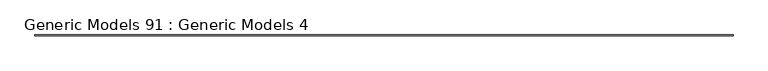
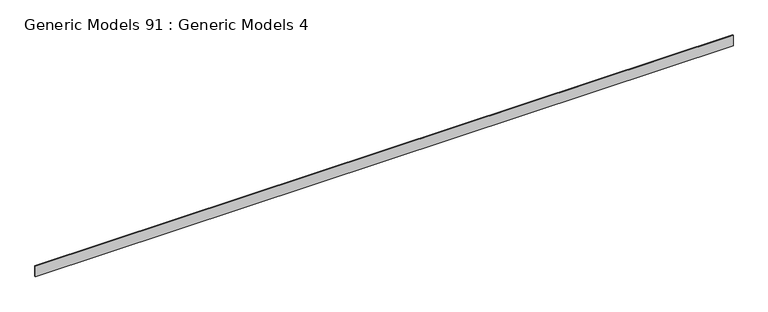
"""IFC4 building model written with IfcOpenShell, lengths in millimetres: proxy geometry, Generic Models 91 : Generic Models 4."""

from ifc_helpers import new_model, si_unit, frame, origin, place, context, project, spatial, polyline, outline, extrude, source, transform, mapped, element, save


def generic_models_91_generic_models_4_9db0eba9(model_context):
    return source(origin(), model_context, "Body", "SweptSolid", [
        extrude(outline(polyline([(-2152.1733045, 51452.647716), (-2152.1733045, 51433.597716), (-20795.7733045, 51433.597716), (-20795.7733045, 51452.647716), (-2152.1733045, 51452.647716)])), frame((0.0, 0.0, 126841.091198), z_axis=(0.0, 0.0, 1.0), x_axis=(1.0, 0.0, 0.0)), (0.0, 0.0, 1.0), 290.0279303),
    ])


if __name__ == "__main__":
    model = new_model("IFC4")
    model_context = context("Model", 3, world=origin())
    ifc_project = project(units=[si_unit("LENGTHUNIT", "METRE", prefix="MILLI")], contexts=[model_context])
    site = spatial("IfcSite", under=ifc_project)
    building = spatial("IfcBuilding", under=site)
    placement = place(None, origin())
    generic_models_91_generic_models_4_shape = generic_models_91_generic_models_4_9db0eba9(model_context)
    element("IfcBuildingElementProxy", 1, Name="Generic Models 91 : Generic Models 4", ObjectType="Generic Models 91 : Generic Models 4", at=placement, inside=building, context=model_context, shape_type="MappedRepresentation", body=[
        mapped(generic_models_91_generic_models_4_shape, transform((0.0, 0.0, 0.0), x_axis=(1.0, 0.0, 0.0), y_axis=(0.0, 1.0, 0.0), z_axis=(0.0, 0.0, 1.0))),
    ])
    save(model, "model.ifc")

# Revit data of these elements
# Element 1 (IfcBuildingElementProxy, "Generic Models 91 : Generic Models 4")
#   Materials on its faces: "_CDX PLYWOOD - SEE STRUCT DWGs"
# Materials
#   "_CDX PLYWOOD - SEE STRUCT DWGs": class "Generic", colour RGB 98 75 74, transparency 0, Cost = 0
